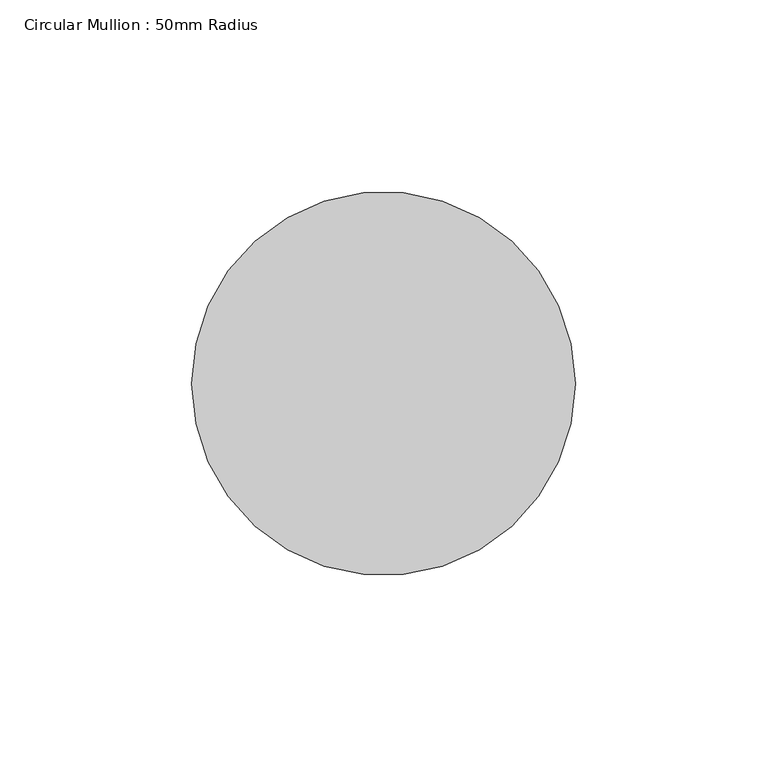
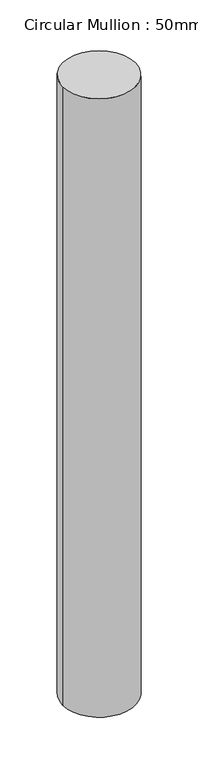
"""IFC4 building model written with IfcOpenShell, lengths in millimetres: member geometry, Circular Mullion : 50mm Radius."""

from ifc_helpers import new_model, si_unit, point, frame, origin, origin_2d, place, context, project, spatial, circle_curve, trimmed, segment, composite_curve, outline, extrude, source, transform, mapped, element, save


def circular_mullion_50mm_radius_42e806ed(model_context):
    return source(origin(), model_context, "Body", "SweptSolid", [
        extrude(outline(composite_curve([segment(trimmed(circle_curve(origin_2d(), 50.0), [point((50.0, 0.0))], [point((-50.0, 0.0))], False, "CARTESIAN"), True, "CONTINUOUS"), segment(trimmed(circle_curve(origin_2d(), 50.0), [point((-50.0, 0.0))], [point((50.0, 0.0))], False, "CARTESIAN"), True, "CONTINUOUS")], self_intersect=False)), frame((0.0, 0.0, -900.0268114), z_axis=(0.0, 0.0, 1.0), x_axis=(1.0, 0.0, 0.0)), (0.0, 0.0, 1.0), 900.0268114),
    ])


if __name__ == "__main__":
    model = new_model("IFC4")
    model_context = context("Model", 3, world=origin())
    ifc_project = project(units=[si_unit("LENGTHUNIT", "METRE", prefix="MILLI")], contexts=[model_context])
    site = spatial("IfcSite", under=ifc_project)
    building = spatial("IfcBuilding", under=site)
    placement = place(None, origin())
    circular_mullion_50mm_radius_shape = circular_mullion_50mm_radius_42e806ed(model_context)
    element("IfcMember", 1, ObjectType="Circular Mullion : 50mm Radius", at=placement, inside=building, context=model_context, shape_type="MappedRepresentation", body=[
        mapped(circular_mullion_50mm_radius_shape, transform((0.0, 0.0, 0.0), x_axis=(1.0, 0.0, 0.0), y_axis=(0.0, 1.0, 0.0), z_axis=(0.0, 0.0, 1.0))),
    ])
    save(model, "model.ifc")

# Revit data of these elements
# Type "Circular Mullion : 50mm Radius"
#   built-in parameter 1007350 = 0.164042 (stored number, unit not read)
# Element 1 (IfcMember, "Circular Mullion : 50mm Radius")
#   Materials on its faces: "Aluminium"
# Materials
#   "Aluminium": class "Metal", colour RGB 247 247 247, transparency 0, Description = "Aluminium 6061", Cost = 0
